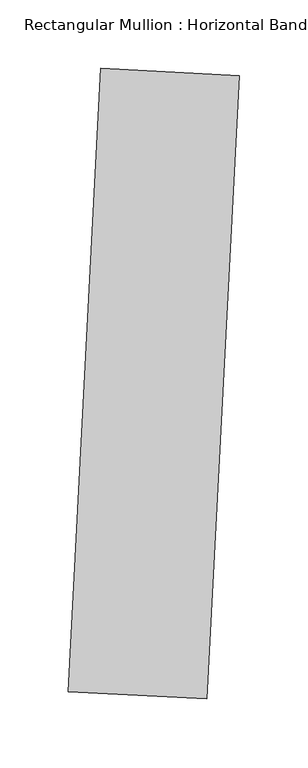
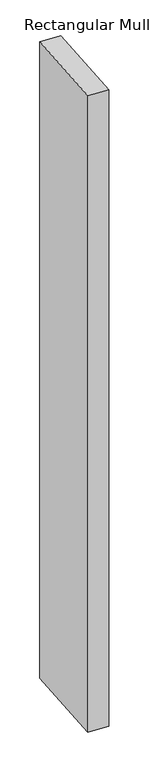
"""IFC4 building model written with IfcOpenShell, lengths in millimetres: member geometry, Rectangular Mullion : Horizontal Band."""

from ifc_helpers import new_model, si_unit, frame, origin, place, context, project, spatial, polyline, outline, extrude, source, transform, mapped, element, save


def rectangular_mullion_horizontal_band_591d7d7b(model_context):
    return source(origin(), model_context, "Body", "SweptSolid", [
        extrude(outline(polyline([(62.69438, 301.8280451), (38.7663808, -154.7453782), (-62.69438, -149.4280451), (-38.7663808, 307.1453782), (62.69438, 301.8280451)])), frame((0.0, 0.0, -3352.8), z_axis=(0.0, 0.0, 1.0), x_axis=(1.0, 0.0, 0.0)), (0.0, 0.0, 1.0), 3352.8),
    ])


if __name__ == "__main__":
    model = new_model("IFC4")
    model_context = context("Model", 3, world=origin())
    ifc_project = project(units=[si_unit("LENGTHUNIT", "METRE", prefix="MILLI")], contexts=[model_context])
    site = spatial("IfcSite", under=ifc_project)
    building = spatial("IfcBuilding", under=site)
    placement = place(None, origin())
    rectangular_mullion_horizontal_band_shape = rectangular_mullion_horizontal_band_591d7d7b(model_context)
    element("IfcMember", 1, ObjectType="Rectangular Mullion : Horizontal Band", at=placement, inside=building, context=model_context, shape_type="MappedRepresentation", body=[
        mapped(rectangular_mullion_horizontal_band_shape, transform((0.0, 0.0, 0.0), x_axis=(1.0, 0.0, 0.0), y_axis=(0.0, 1.0, 0.0), z_axis=(0.0, 0.0, 1.0))),
    ])
    save(model, "model.ifc")

# Revit data of these elements
# Type "Rectangular Mullion : Horizontal Band"
#   built-in parameter 1007351 = 0.25 (stored number, unit not read)
#   built-in parameter 1007304 = 1.5 (stored number, unit not read)
#   built-in parameter 1007301 = 0.166667 (stored number, unit not read)
#   built-in parameter 1007300 = 0.166667 (stored number, unit not read)
# Element 1 (IfcMember, "Rectangular Mullion : Horizontal Band")
#   Materials on its faces: "Aluminum"
# Materials
#   "Aluminum": class "Metal", colour RGB 247 247 247, transparency 0, Description = "Aluminum 6061", Cost = 0
